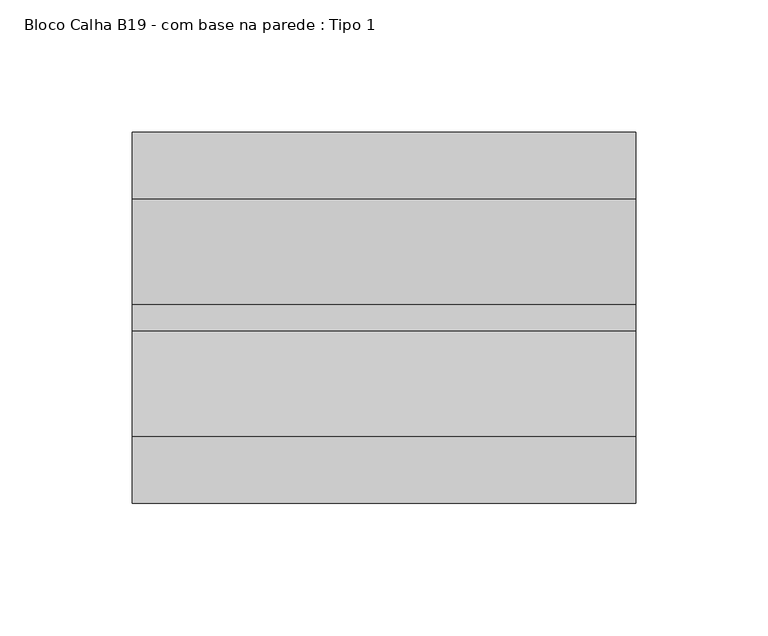
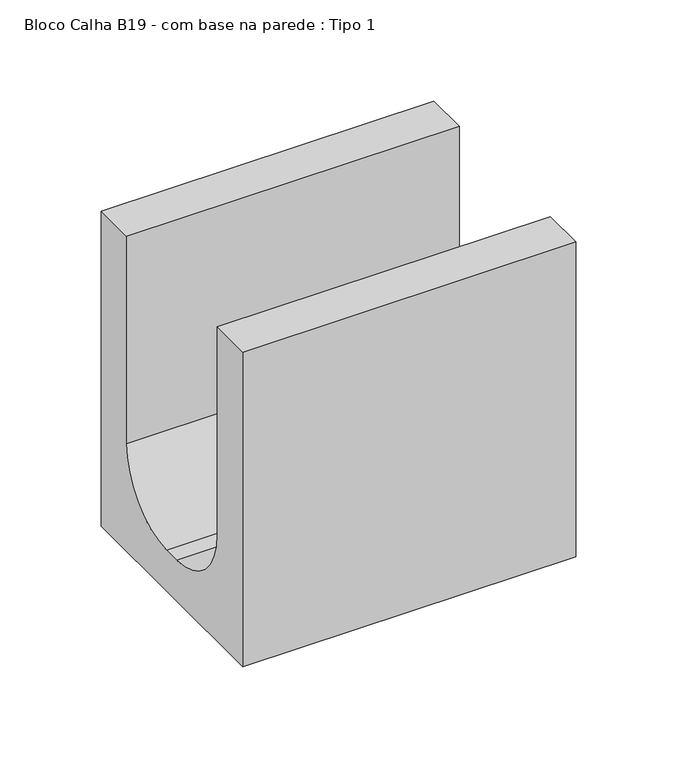
"""IFC4 building model written with IfcOpenShell, lengths in millimetres: proxy geometry, Bloco Calha B19 - com base na parede : Tipo 1."""

import ifcopenshell
import ifcopenshell.guid

model = None  # the IFC model being written
_history = None  # IfcOwnerHistory: only IFC2X3 demands one
_inside = {}  # id of a spatial element -> (the spatial element, [elements in it])
_under = {}  # id of a project, library or spatial element -> (it, [spatial elements below it])
_declared = {}  # id of a project -> (the project, [libraries it declares])
_typed = {}  # id of a type object -> (the type object, [elements of that type])
_made_of = {}  # id of a material, layer set ... -> (it, [elements and type objects made of it])


def new_model(schema):
    """Start an empty IFC model of exactly this schema.

    Asked for "IFC4X3", IfcOpenShell would pick the latest addendum, in which some entities
    have other attributes; the version numbers below select the first issue.
    IFC2X3 requires an IfcOwnerHistory on every rooted entity: one is made here for all.
    """
    global model, _history
    if schema == "IFC4X3":
        model = ifcopenshell.file(schema_version=(4, 3, 0, 0))
    else:
        model = ifcopenshell.file(schema=schema)
    _inside.clear()
    _under.clear()
    _declared.clear()
    _typed.clear()
    _made_of.clear()
    _history = None
    if model.schema == "IFC2X3":
        org = make("IfcOrganization", Name="unknown")
        user = make(
            "IfcPersonAndOrganization",
            ThePerson=make("IfcPerson", FamilyName="unknown"),
            TheOrganization=org,
        )
        app = make(
            "IfcApplication",
            ApplicationDeveloper=org,
            Version="unknown",
            ApplicationFullName="unknown",
            ApplicationIdentifier="unknown",
        )
        _history = make(
            "IfcOwnerHistory",
            OwningUser=user,
            OwningApplication=app,
            ChangeAction="ADDED",
            CreationDate=0,
        )
    return model


def make(cls, **values):
    """One entity of the class cls with the attributes given. An attribute that is None is left unset."""
    return model.create_entity(
        cls, **{name: value for name, value in values.items() if value is not None}
    )


def rooted(cls, **values):
    """An entity with a GlobalId (a new one), such as an element, a storey or a relation."""
    return make(cls, GlobalId=ifcopenshell.guid.new(), OwnerHistory=_history, **values)


def si_unit(unit_type, name, prefix=None):
    """IfcSIUnit, for example si_unit("LENGTHUNIT", "METRE", prefix="MILLI")."""
    return make("IfcSIUnit", UnitType=unit_type, Prefix=prefix, Name=name)


def assignment(units):
    """IfcUnitAssignment: the units of a project."""
    return None if units is None else make("IfcUnitAssignment", Units=units)


def point(xyz):
    """IfcCartesianPoint."""
    return None if xyz is None else make("IfcCartesianPoint", Coordinates=xyz)


def direction(xyz):
    """IfcDirection."""
    return None if xyz is None else make("IfcDirection", DirectionRatios=xyz)


def frame(location, z_axis=None, x_axis=None):
    """IfcAxis2Placement3D, a coordinate frame: its origin and axes. An axis left out is left unset."""
    return make(
        "IfcAxis2Placement3D",
        Location=point(location),
        Axis=direction(z_axis),
        RefDirection=direction(x_axis),
    )


def frame_2d(location, x_axis=None):
    """IfcAxis2Placement2D, a coordinate frame in the plane: its origin and x axis."""
    return make(
        "IfcAxis2Placement2D", Location=point(location), RefDirection=direction(x_axis)
    )


def origin():
    """The frame at (0, 0, 0) with its axes left unset."""
    return frame((0.0, 0.0, 0.0))


def place(relative_to, where):
    """IfcLocalPlacement: puts the frame where relative to a parent placement (None: the world)."""
    return make(
        "IfcLocalPlacement", PlacementRelTo=relative_to, RelativePlacement=where
    )


def context(
    kind, dimensions, precision=None, world=None, true_north=None, identifier=None
):
    """IfcGeometricRepresentationContext, for example the 3D "Model" context."""
    return make(
        "IfcGeometricRepresentationContext",
        ContextIdentifier=identifier,
        ContextType=kind,
        CoordinateSpaceDimension=dimensions,
        Precision=precision,
        WorldCoordinateSystem=world,
        TrueNorth=true_north,
    )


def project(units=None, contexts=None):
    """IfcProject with its units and contexts."""
    return rooted(
        "IfcProject",
        Name="project",
        RepresentationContexts=contexts,
        UnitsInContext=assignment(units),
    )


def spatial(cls, under=None, at=None, **own):
    """A site, building, storey or space (cls), placed at a placement, below another one or the project."""
    s = rooted(cls, ObjectPlacement=at, **own)
    if under is not None:
        _under.setdefault(under.id(), (under, []))[1].append(s)
    return s


def polyline(points):
    """IfcPolyline through the points."""
    return make("IfcPolyline", Points=[point(p) for p in points])


def circle_curve(where, radius):
    """IfcCircle in the frame where."""
    return make("IfcCircle", Position=where, Radius=radius)


def trimmed(basis, trim1, trim2, sense, master):
    """IfcTrimmedCurve: the piece of a basis curve between two trims."""
    return make(
        "IfcTrimmedCurve",
        BasisCurve=basis,
        Trim1=trim1,
        Trim2=trim2,
        SenseAgreement=sense,
        MasterRepresentation=master,
    )


def segment(curve, same_sense, transition):
    """IfcCompositeCurveSegment."""
    return make(
        "IfcCompositeCurveSegment",
        Transition=transition,
        SameSense=same_sense,
        ParentCurve=curve,
    )


def composite_curve(segments, self_intersect=None):
    """IfcCompositeCurve: segments joined end to end."""
    return make("IfcCompositeCurve", Segments=segments, SelfIntersect=self_intersect)


def outline(outer, holes=None, kind="AREA"):
    """IfcArbitraryClosedProfileDef: a profile drawn as a closed curve; with holes, ...WithVoids."""
    if holes is None:
        return make("IfcArbitraryClosedProfileDef", ProfileType=kind, OuterCurve=outer)
    return make(
        "IfcArbitraryProfileDefWithVoids",
        ProfileType=kind,
        OuterCurve=outer,
        InnerCurves=holes,
    )


def extrude(swept, where, along, depth):
    """IfcExtrudedAreaSolid: the profile swept, set in the frame where, extruded along a direction by depth."""
    return make(
        "IfcExtrudedAreaSolid",
        SweptArea=swept,
        Position=where,
        ExtrudedDirection=direction(along),
        Depth=depth,
    )


def shape(context_of_items, identifier, shape_type, items):
    """IfcShapeRepresentation: the items that make up one representation, for example the "Body"."""
    return make(
        "IfcShapeRepresentation",
        ContextOfItems=context_of_items,
        RepresentationIdentifier=identifier,
        RepresentationType=shape_type,
        Items=items,
    )


def source(mapping_origin, context_of_items, identifier, shape_type, items):
    """IfcRepresentationMap: a shape defined once, which mapped items show again and again."""
    return make(
        "IfcRepresentationMap",
        MappingOrigin=mapping_origin,
        MappedRepresentation=shape(context_of_items, identifier, shape_type, items),
    )


def transform(
    local_origin,
    x_axis=None,
    y_axis=None,
    z_axis=None,
    scale=None,
    scale2=None,
    scale3=None,
    uniform=True,
):
    """IfcCartesianTransformationOperator3D, or its non-uniform kind. x_axis, y_axis, z_axis: its Axis1, 2, 3."""
    if uniform:
        return make(
            "IfcCartesianTransformationOperator3D",
            Axis1=direction(x_axis),
            Axis2=direction(y_axis),
            LocalOrigin=point(local_origin),
            Scale=scale,
            Axis3=direction(z_axis),
        )
    return make(
        "IfcCartesianTransformationOperator3DnonUniform",
        Axis1=direction(x_axis),
        Axis2=direction(y_axis),
        LocalOrigin=point(local_origin),
        Scale=scale,
        Axis3=direction(z_axis),
        Scale2=scale2,
        Scale3=scale3,
    )


def mapped(mapping_source, mapping_target):
    """IfcMappedItem: shows the shape of a source again, moved by a transform."""
    return make(
        "IfcMappedItem", MappingSource=mapping_source, MappingTarget=mapping_target
    )


def made_of(thing, what):
    """Note that an element or type object is made of a material, layer set ...; save() writes the relation."""
    if what is not None:
        _made_of.setdefault(what.id(), (what, []))[1].append(thing)
    return thing


def element(
    cls,
    number,
    at=None,
    inside=None,
    cuts=None,
    type_object=None,
    material=None,
    context=None,
    identifier="Body",
    shape_type=None,
    held_by="IfcProductDefinitionShape",
    body=None,
    shapes=None,
    **own,
):
    """One element of the class cls, such as IfcWall. Its Tag is "e" and its number.

    at: its placement. inside: the storey or other place that contains it. cuts: it is an
    opening in that element (IfcRelVoidsElement). A single representation is given by context,
    identifier, shape_type and body (its items); several are given by shapes. held_by: the class
    of the entity that holds the representations. save() writes the other relations.
    """
    e = rooted(cls, Tag="e%d" % number, ObjectPlacement=at, **own)
    if body is not None:
        shapes = [shape(context, identifier, shape_type, body)]
    if shapes is not None:
        e.Representation = make(held_by, Representations=shapes)
    if inside is not None:
        _inside.setdefault(inside.id(), (inside, []))[1].append(e)
    if cuts is not None:
        rooted(
            "IfcRelVoidsElement", RelatingBuildingElement=cuts, RelatedOpeningElement=e
        )
    if type_object is not None:
        _typed.setdefault(type_object.id(), (type_object, []))[1].append(e)
    return made_of(e, material)


def aggregate(whole, parts):
    """IfcRelAggregates: a whole, such as a stair, and the parts it consists of."""
    return rooted("IfcRelAggregates", RelatingObject=whole, RelatedObjects=parts)


def save(model, path):
    """Write the relations noted so far, then the file.

    IfcRelAggregates (storeys below a building ...), IfcRelContainedInSpatialStructure (elements
    in a storey), IfcRelDefinesByType, IfcRelAssociatesMaterial and IfcRelDeclares: one each for
    every whole, place, type object, material and project.
    """
    for whole, parts in _under.values():
        aggregate(whole, parts)
    for where, things in _inside.values():
        rooted(
            "IfcRelContainedInSpatialStructure",
            RelatedElements=things,
            RelatingStructure=where,
        )
    for kind, things in _typed.values():
        rooted("IfcRelDefinesByType", RelatedObjects=things, RelatingType=kind)
    for what, things in _made_of.values():
        rooted("IfcRelAssociatesMaterial", RelatedObjects=things, RelatingMaterial=what)
    for by, libraries in _declared.values():
        rooted("IfcRelDeclares", RelatingContext=by, RelatedDefinitions=libraries)
    model.write(path)


def bloco_calha_b19_com_base_na_parede_tipo_1_535c7f08(model_context):
    return source(origin(), model_context, "Body", "SweptSolid", [
        extrude(outline(composite_curve([segment(polyline([(70.0, 0.0), (-70.0, 0.0), (-70.0, 190.0), (-45.0, 190.0), (-45.0, 65.0)]), True, "CONTINUOUS"), segment(trimmed(circle_curve(frame_2d((-5.0, 65.0)), 40.0), [point((-45.0, 65.0))], [point((-5.0, 25.0))], True, "CARTESIAN"), True, "CONTINUOUS"), segment(polyline([(-5.0, 25.0), (5.0, 25.0)]), True, "CONTINUOUS"), segment(trimmed(circle_curve(frame_2d((5.0, 65.0)), 40.0), [point((5.0, 25.0))], [point((45.0, 65.0))], True, "CARTESIAN"), True, "CONTINUOUS"), segment(polyline([(45.0, 65.0), (45.0, 190.0), (70.0, 190.0), (70.0, 0.0)]), True, "CONTINUOUS")], self_intersect=False)), frame((30.0, 0.0, 0.0), z_axis=(1.0, 0.0, 0.0), x_axis=(0.0, 1.0, 0.0)), (0.0, 0.0, 1.0), 190.0),
    ])


if __name__ == "__main__":
    model = new_model("IFC4")
    model_context = context("Model", 3, world=origin())
    ifc_project = project(units=[si_unit("LENGTHUNIT", "METRE", prefix="MILLI")], contexts=[model_context])
    site = spatial("IfcSite", under=ifc_project)
    building = spatial("IfcBuilding", under=site)
    placement = place(None, origin())
    bloco_calha_b19_com_base_na_parede_tipo_1_shape = bloco_calha_b19_com_base_na_parede_tipo_1_535c7f08(model_context)
    element("IfcBuildingElementProxy", 1, Name="Bloco Calha B19 - com base na parede : Tipo 1", ObjectType="Bloco Calha B19 - com base na parede : Tipo 1", at=placement, inside=building, context=model_context, shape_type="MappedRepresentation", body=[
        mapped(bloco_calha_b19_com_base_na_parede_tipo_1_shape, transform((0.0, 0.0, 0.0), x_axis=(1.0, 0.0, 0.0), y_axis=(0.0, 1.0, 0.0), z_axis=(0.0, 0.0, 1.0))),
    ])
    save(model, "model.ifc")

# Revit data of these elements
# Type "Bloco Calha B19 - com base na parede : Tipo 1"
#   SINAPI = ""
#   Assembly Code = ""
